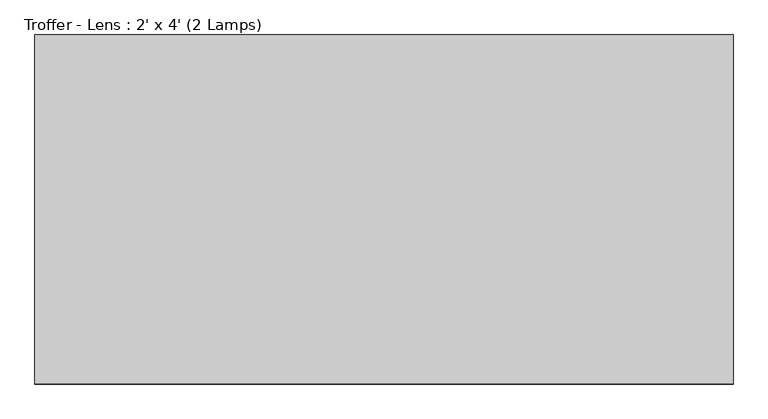
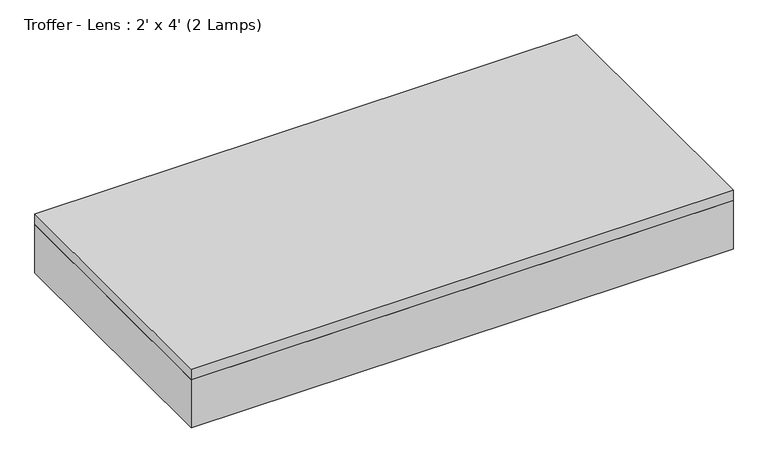
"""IFC4 building model written with IfcOpenShell, lengths in millimetres: light fixture geometry, Troffer - Lens : 2' x 4' (2 Lamps)."""

from ifc_helpers import new_model, si_unit, frame, origin, place, context, project, spatial, polyline, outline, extrude, source, transform, mapped, element, save


def troffer_lens_2_x_4_2_lamps_b3407adc(model_context):
    return source(origin(), model_context, "Body", "SweptSolid", [
        extrude(outline(polyline([(565.4964984, 219.9340679), (565.4964984, -338.8659321), (-602.9035016, -338.8659321), (-602.9035016, 219.9340679), (565.4964984, 219.9340679)])), frame((0.0, 0.0, 2438.4), z_axis=(0.0, 0.0, 1.0), x_axis=(1.0, 0.0, 0.0)), (0.0, 0.0, 1.0), 6.35),
        extrude(outline(polyline([(590.8964984, 245.3340679), (590.8964984, -364.2659321), (-628.3035016, -364.2659321), (-628.3035016, 245.3340679), (590.8964984, 245.3340679)]), holes=[polyline([(565.4964984, 219.9340679), (-602.9035016, 219.9340679), (-602.9035016, -338.8659321), (565.4964984, -338.8659321), (565.4964984, 219.9340679)])]), frame((0.0, 0.0, 2438.4), z_axis=(0.0, 0.0, 1.0), x_axis=(1.0, 0.0, 0.0)), (0.0, 0.0, 1.0), 114.3),
        extrude(outline(polyline([(590.8964984, 245.3340679), (590.8964984, -364.2659321), (-628.3035016, -364.2659321), (-628.3035016, 245.3340679), (590.8964984, 245.3340679)])), frame((0.0, 0.0, 2552.7), z_axis=(0.0, 0.0, 1.0), x_axis=(1.0, 0.0, 0.0)), (0.0, 0.0, 1.0), 25.4),
    ])


if __name__ == "__main__":
    model = new_model("IFC4")
    model_context = context("Model", 3, world=origin())
    ifc_project = project(units=[si_unit("LENGTHUNIT", "METRE", prefix="MILLI")], contexts=[model_context])
    site = spatial("IfcSite", under=ifc_project)
    building = spatial("IfcBuilding", under=site)
    placement = place(None, origin())
    troffer_lens_2_x_4_2_lamps_shape = troffer_lens_2_x_4_2_lamps_b3407adc(model_context)
    element("IfcLightFixture", 1, ObjectType="Troffer - Lens : 2' x 4' (2 Lamps)", at=placement, inside=building, context=model_context, shape_type="MappedRepresentation", body=[
        mapped(troffer_lens_2_x_4_2_lamps_shape, transform((0.0, 0.0, 0.0), x_axis=(1.0, 0.0, 0.0), y_axis=(0.0, 1.0, 0.0), z_axis=(0.0, 0.0, 1.0))),
    ])
    save(model, "model.ifc")

# Revit data of these elements
# Type "Troffer - Lens : 2' x 4' (2 Lamps)"
#   Assembly Code = "D5020210"
#   Lamp = "T-12"
#   Wattage Comments = "(2)20"
#   Wattage = 16.1571 W
#   built-in parameter 1150110 = 1 (stored number, unit not read)
#   built-in parameter 1114217 = 1 (stored number, unit not read)
#   built-in parameter 1150109 = 1 (stored number, unit not read)
#   built-in parameter 1150113 = 1 (stored number, unit not read)
#   built-in parameter 1150105 = 190.986 (stored number, unit not read)
#   built-in parameter 1150115 = 1 (stored number, unit not read)
#   Light Source Symbol Size = 2' - 0"
#   built-in parameter 1150112 = 1 (stored number, unit not read)
#   built-in parameter 1150114 = 1 (stored number, unit not read)
#   built-in parameter 1150107 = 3200 (stored number, unit not read)
#   built-in parameter 1150106 = 1.90986 (stored number, unit not read)
#   Emit from Line Length = 3' - 10"
#   built-in parameter 1150104 = 13.8 (stored number, unit not read)
#   built-in parameter 1114218 = 1 (stored number, unit not read)
#   built-in parameter 1150133 = 10 (stored number, unit not read)
#   Circle Diameter = 1' - 2.4"
#   Length = 4' - 0"
#   Lumens = 2400 lm
#   Width = 2' - 0"
#   built-in parameter 1150134 = 3
#   built-in parameter 1150132 = 2
#   Color Filter = 16777215
#   Diffuser = none
#   Light Box = none
#   Dimming Lamp Color Temperature Shift = (empty or 0)
